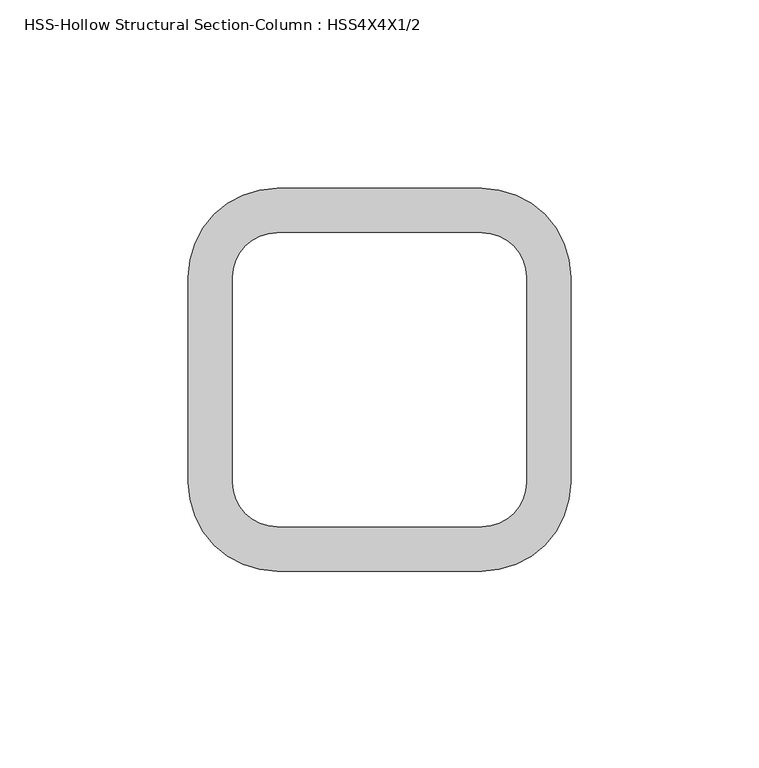
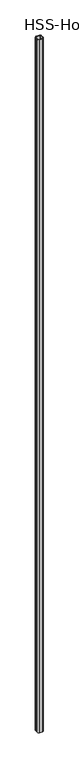
"""IFC4 building model written with IfcOpenShell, lengths in millimetres: column geometry, HSS-Hollow Structural Section-Column : HSS4X4X1/2."""

from ifc_helpers import new_model, si_unit, point, frame, frame_2d, origin, place, context, project, spatial, polyline, circle_curve, trimmed, segment, composite_curve, outline, extrude, source, transform, mapped, element, save


def hss_hollow_structural_section_column_hss4x4x1_2_02489a23(model_context):
    return source(origin(), model_context, "Body", "SweptSolid", [
        extrude(outline(composite_curve([segment(trimmed(circle_curve(frame_2d((27.178, 27.178)), 23.622), [point((27.178, 50.8))], [point((50.8, 27.178))], False, "CARTESIAN"), True, "CONTINUOUS"), segment(polyline([(50.8, 27.178), (50.8, -27.178)]), True, "CONTINUOUS"), segment(trimmed(circle_curve(frame_2d((27.178, -27.178)), 23.622), [point((50.8, -27.178))], [point((27.178, -50.8))], False, "CARTESIAN"), True, "CONTINUOUS"), segment(polyline([(27.178, -50.8), (-27.178, -50.8)]), True, "CONTINUOUS"), segment(trimmed(circle_curve(frame_2d((-27.178, -27.178)), 23.622), [point((-27.178, -50.8))], [point((-50.8, -27.178))], False, "CARTESIAN"), True, "CONTINUOUS"), segment(polyline([(-50.8, -27.178), (-50.8, 27.178)]), True, "CONTINUOUS"), segment(trimmed(circle_curve(frame_2d((-27.178, 27.178)), 23.622), [point((-50.8, 27.178))], [point((-27.178, 50.8))], False, "CARTESIAN"), True, "CONTINUOUS"), segment(polyline([(-27.178, 50.8), (27.178, 50.8)]), True, "CONTINUOUS")], self_intersect=False), holes=[composite_curve([segment(polyline([(27.178, 38.989), (-27.178, 38.989)]), True, "CONTINUOUS"), segment(trimmed(circle_curve(frame_2d((-27.178, 27.178)), 11.811), [point((-27.178, 38.989))], [point((-38.989, 27.178))], True, "CARTESIAN"), True, "CONTINUOUS"), segment(polyline([(-38.989, 27.178), (-38.989, -27.178)]), True, "CONTINUOUS"), segment(trimmed(circle_curve(frame_2d((-27.178, -27.178)), 11.811), [point((-38.989, -27.178))], [point((-27.178, -38.989))], True, "CARTESIAN"), True, "CONTINUOUS"), segment(polyline([(-27.178, -38.989), (27.178, -38.989)]), True, "CONTINUOUS"), segment(trimmed(circle_curve(frame_2d((27.178, -27.178)), 11.811), [point((27.178, -38.989))], [point((38.989, -27.178))], True, "CARTESIAN"), True, "CONTINUOUS"), segment(polyline([(38.989, -27.178), (38.989, 27.178)]), True, "CONTINUOUS"), segment(trimmed(circle_curve(frame_2d((27.178, 27.178)), 11.811), [point((38.989, 27.178))], [point((27.178, 38.989))], True, "CARTESIAN"), True, "CONTINUOUS")], self_intersect=False)]), frame((0.0, 0.0, -609.6), z_axis=(0.0, 0.0, 1.0), x_axis=(1.0, 0.0, 0.0)), (0.0, 0.0, 1.0), 12954.0),
    ])


if __name__ == "__main__":
    model = new_model("IFC4")
    model_context = context("Model", 3, world=origin())
    ifc_project = project(units=[si_unit("LENGTHUNIT", "METRE", prefix="MILLI")], contexts=[model_context])
    site = spatial("IfcSite", under=ifc_project)
    building = spatial("IfcBuilding", under=site)
    placement = place(None, origin())
    hss_hollow_structural_section_column_hss4x4x1_2_shape = hss_hollow_structural_section_column_hss4x4x1_2_02489a23(model_context)
    element("IfcColumn", 1, ObjectType="HSS-Hollow Structural Section-Column : HSS4X4X1/2", at=placement, inside=building, context=model_context, shape_type="MappedRepresentation", body=[
        mapped(hss_hollow_structural_section_column_hss4x4x1_2_shape, transform((0.0, 0.0, 0.0), x_axis=(1.0, 0.0, 0.0), y_axis=(0.0, 1.0, 0.0), z_axis=(0.0, 0.0, 1.0))),
    ])
    save(model, "model.ifc")

# Revit data of these elements
# Type "HSS-Hollow Structural Section-Column : HSS4X4X1/2"
#   Assembly Code = "B10"
#   Shape = "Square"
#   W = 21.5
#   Ht = 0' - 4"
#   b = 0' - 4"
#   kr = 0' - 0.93"
#   t = 0' - 0.465"
#   A = 0.0418056 SF
#   Structural Material [instance default] = Steel ASTM A500, Grade B, Rectangular and Square
# Element 1 (IfcColumn, "HSS-Hollow Structural Section-Column : HSS4X4X1/2")
#   Materials on its faces: "Steel ASTM A500, Grade B, Rectangular and Square"
# Materials
#   "Steel ASTM A500, Grade B, Rectangular and Square": class "Metal", colour RGB 199 199 199, transparency 0, Description = "Carbon steel", Cost = 0
